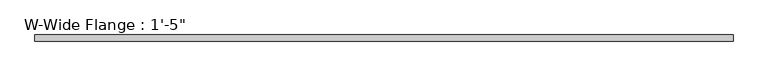
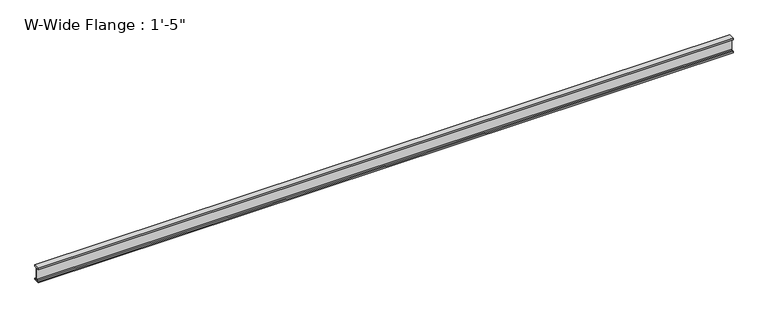
"""IFC4 building model written with IfcOpenShell, lengths in millimetres: beam geometry."""

from ifc_helpers import new_model, si_unit, point, frame, frame_2d, origin, place, context, project, spatial, polyline, circle_curve, trimmed, segment, composite_curve, outline, extrude, source, transform, mapped, element, save


def beam_58e5e3b7(model_context):
    return source(origin(), model_context, "Body", "SweptSolid", [
        extrude(outline(composite_curve([segment(polyline([(76.2, -155.956), (76.2, -190.5), (-76.2, -190.5), (-76.2, -155.956), (-32.131, -155.956)]), True, "CONTINUOUS"), segment(trimmed(circle_curve(frame_2d((-32.131, -133.35)), 22.606), [point((-32.131, -155.956))], [point((-9.525, -133.35))], True, "CARTESIAN"), True, "CONTINUOUS"), segment(polyline([(-9.525, -133.35), (-9.525, 133.35)]), True, "CONTINUOUS"), segment(trimmed(circle_curve(frame_2d((-32.131, 133.35)), 22.606), [point((-9.525, 133.35))], [point((-32.131, 155.956))], True, "CARTESIAN"), True, "CONTINUOUS"), segment(polyline([(-32.131, 155.956), (-76.2, 155.956), (-76.2, 190.5), (76.2, 190.5), (76.2, 155.956), (32.131, 155.956)]), True, "CONTINUOUS"), segment(trimmed(circle_curve(frame_2d((32.131, 133.35)), 22.606), [point((32.131, 155.956))], [point((9.525, 133.35))], True, "CARTESIAN"), True, "CONTINUOUS"), segment(polyline([(9.525, 133.35), (9.525, -133.35)]), True, "CONTINUOUS"), segment(trimmed(circle_curve(frame_2d((32.131, -133.35)), 22.606), [point((9.525, -133.35))], [point((32.131, -155.956))], True, "CARTESIAN"), True, "CONTINUOUS"), segment(polyline([(32.131, -155.956), (76.2, -155.956)]), True, "CONTINUOUS")], self_intersect=False)), frame((-8558.576002, 0.0, 0.0), z_axis=(1.0, 0.0, 0.0), x_axis=(0.0, 1.0, 0.0)), (0.0, 0.0, 1.0), 17399.288347),
    ])


if __name__ == "__main__":
    model = new_model("IFC4")
    model_context = context("Model", 3, world=origin())
    ifc_project = project(units=[si_unit("LENGTHUNIT", "METRE", prefix="MILLI")], contexts=[model_context])
    site = spatial("IfcSite", under=ifc_project)
    building = spatial("IfcBuilding", under=site)
    placement = place(None, origin())
    beam_shape = beam_58e5e3b7(model_context)
    element("IfcBeam", 1, ObjectType="W-Wide Flange : 1'-5\"", at=placement, inside=building, context=model_context, shape_type="MappedRepresentation", body=[
        mapped(beam_shape, transform((0.0, 0.0, 0.0), x_axis=(1.0, 0.0, 0.0), y_axis=(0.0, 1.0, 0.0), z_axis=(0.0, 0.0, 1.0))),
    ])
    save(model, "model.ifc")

# Revit data of these elements
# Type "W-Wide Flange : 1'-5\""
#   Assembly Code = "B10"
#   W = 166
#   Length [instance default] = 5' - 0"
#   bf = 0' - 6"
#   d = 1' - 3"
#   k = 0' - 2 1/4"
#   k2 = 0' - 0.89"
#   tf = 0' - 1.36"
#   tw = 0' - 0 3/4"
#   A = 0.338889 SF
#   Structural Material [instance default] = Steel ASTM A992
# Element 1 (IfcBeam, "W-Wide Flange : 1'-5\"")
#   Structural Material = STRUCTURAL STEEL - SEE STRUCT. DWGS
#   Materials on its faces: "STRUCTURAL STEEL - SEE STRUCT. DWGS"
# Materials
#   "Steel ASTM A992": class "Metal", colour RGB 199 199 199, transparency 0, Description = "Structural steel 50ksi", Cost = 0
#   "STRUCTURAL STEEL - SEE STRUCT. DWGS": class "Metal", colour RGB 137 146 153, transparency 0, Description = "Steel, mill finish", Cost = 0
